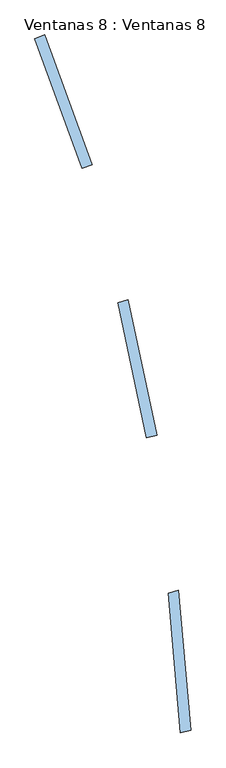
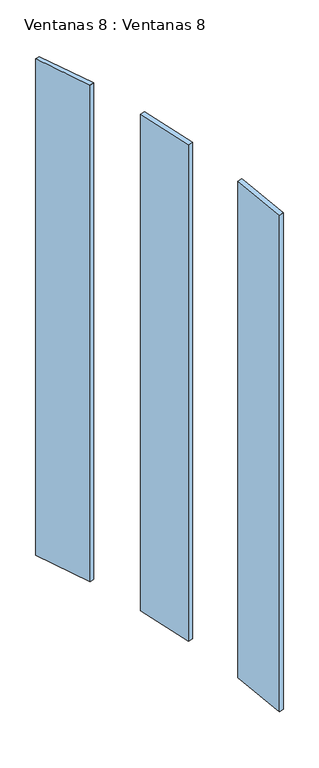
"""IFC4 building model written with IfcOpenShell, lengths in millimetres: window geometry, Ventanas 8 : Ventanas 8."""

from ifc_helpers import new_model, si_unit, frame, origin, place, context, project, spatial, polyline, outline, extrude, source, transform, mapped, element, save


def ventanas_8_ventanas_8_c419d356(model_context):
    return source(origin(), model_context, "Body", "SweptSolid", [
        extrude(outline(polyline([(6147.143523, 4516.9430054), (6128.3496706, 4510.1026026), (6039.4244333, 4754.422684), (6058.2182857, 4761.2630868), (6147.143523, 4516.9430054)])), frame((0.0, 0.0, 5400.0), z_axis=(0.0, 0.0, 1.0), x_axis=(1.0, 0.0, 0.0)), (0.0, 0.0, 1.0), 2214.4258331),
        extrude(outline(polyline([(6269.4539241, 4007.8274654), (6250.1354076, 4002.6510845), (6196.004183, 4257.3184735), (6215.3226996, 4262.4948544), (6269.4539241, 4007.8274654)])), frame((0.0, 0.0, 5400.0), z_axis=(0.0, 0.0, 1.0), x_axis=(1.0, 0.0, 0.0)), (0.0, 0.0, 1.0), 2214.4258331),
        extrude(outline(polyline([(6333.5911504, 3452.1862494), (6314.2726338, 3447.0098685), (6291.2625661, 3710.0161463), (6310.5810826, 3715.1925272), (6333.5911504, 3452.1862494)])), frame((0.0, 0.0, 5400.0), z_axis=(0.0, 0.0, 1.0), x_axis=(1.0, 0.0, 0.0)), (0.0, 0.0, 1.0), 2214.4258331),
    ])


if __name__ == "__main__":
    model = new_model("IFC4")
    model_context = context("Model", 3, world=origin())
    ifc_project = project(units=[si_unit("LENGTHUNIT", "METRE", prefix="MILLI")], contexts=[model_context])
    site = spatial("IfcSite", under=ifc_project)
    building = spatial("IfcBuilding", under=site)
    placement = place(None, origin())
    ventanas_8_ventanas_8_shape = ventanas_8_ventanas_8_c419d356(model_context)
    element("IfcWindow", 1, ObjectType="Ventanas 8 : Ventanas 8", at=placement, inside=building, context=model_context, shape_type="MappedRepresentation", body=[
        mapped(ventanas_8_ventanas_8_shape, transform((0.0, 0.0, 0.0), x_axis=(1.0, 0.0, 0.0), y_axis=(0.0, 1.0, 0.0), z_axis=(0.0, 0.0, 1.0))),
    ])
    save(model, "model.ifc")

# Revit data of these elements
# Type "Ventanas 8 : Ventanas 8"
#   Type Mark = "34"
# Element 1 (IfcWindow, "Ventanas 8 : Ventanas 8")
#   Materials on its faces: "VIDRIO"
# Materials
#   "VIDRIO": class "Genérico", colour RGB 120 120 120, transparency 0, Cost = 0
